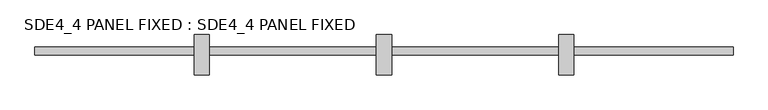
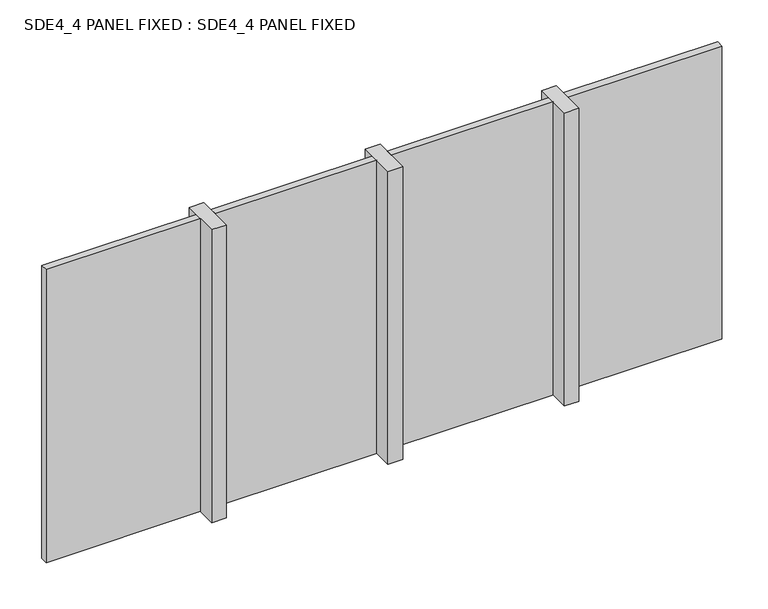
"""IFC4 building model written with IfcOpenShell, lengths in millimetres: plate geometry, SDE4_4 PANEL FIXED : SDE4_4 PANEL FIXED."""

from ifc_helpers import new_model, si_unit, origin, origin_with_axes, place, context, project, spatial, polyline, outline, extrude, source, transform, mapped, element, save


def sde4_4_panel_fixed_sde4_4_panel_fixed_a4a4073a(model_context):
    return source(origin(), model_context, "Body", "SweptSolid", [
        extrude(outline(polyline([(-1150.0, 132.5), (-1150.0, -132.5), (-1250.0, -132.5), (-1250.0, 132.5), (-1150.0, 132.5)])), origin_with_axes(), (0.0, 0.0, 1.0), 2110.0),
        extrude(outline(polyline([(50.0, 132.5), (50.0, -132.5), (-50.0, -132.5), (-50.0, 132.5), (50.0, 132.5)])), origin_with_axes(), (0.0, 0.0, 1.0), 2110.0),
        extrude(outline(polyline([(1250.0, 132.5), (1250.0, -132.5), (1150.0, -132.5), (1150.0, 132.5), (1250.0, 132.5)])), origin_with_axes(), (0.0, 0.0, 1.0), 2110.0),
        extrude(outline(polyline([(2299.0, 50.0), (2299.0, 0.0), (1250.0, 0.0), (1250.0, 50.0), (2299.0, 50.0)])), origin_with_axes(), (0.0, 0.0, 1.0), 2110.0),
        extrude(outline(polyline([(1150.0, 50.0), (1150.0, 0.0), (50.0, 0.0), (50.0, 50.0), (1150.0, 50.0)])), origin_with_axes(), (0.0, 0.0, 1.0), 2110.0),
        extrude(outline(polyline([(-50.0, 50.0), (-50.0, 0.0), (-1150.0, 0.0), (-1150.0, 50.0), (-50.0, 50.0)])), origin_with_axes(), (0.0, 0.0, 1.0), 2110.0),
        extrude(outline(polyline([(-1250.0, 50.0), (-1250.0, 0.0), (-2300.0, 0.0), (-2300.0, 50.0), (-1250.0, 50.0)])), origin_with_axes(), (0.0, 0.0, 1.0), 2110.0),
    ])


if __name__ == "__main__":
    model = new_model("IFC4")
    model_context = context("Model", 3, world=origin())
    ifc_project = project(units=[si_unit("LENGTHUNIT", "METRE", prefix="MILLI")], contexts=[model_context])
    site = spatial("IfcSite", under=ifc_project)
    building = spatial("IfcBuilding", under=site)
    placement = place(None, origin())
    sde4_4_panel_fixed_sde4_4_panel_fixed_shape = sde4_4_panel_fixed_sde4_4_panel_fixed_a4a4073a(model_context)
    element("IfcPlate", 1, ObjectType="SDE4_4 PANEL FIXED : SDE4_4 PANEL FIXED", at=placement, inside=building, context=model_context, shape_type="MappedRepresentation", body=[
        mapped(sde4_4_panel_fixed_sde4_4_panel_fixed_shape, transform((0.0, 0.0, 0.0), x_axis=(1.0, 0.0, 0.0), y_axis=(0.0, 1.0, 0.0), z_axis=(0.0, 0.0, 1.0))),
    ])
    save(model, "model.ifc")

# Revit data of these elements
# Type "SDE4_4 PANEL FIXED : SDE4_4 PANEL FIXED"
#   Type Mark = "CW-GLASS"
#   Analytic Construction = "<None>"
#   Glass = Glass
#   Frame = Aluminium
# Element 1 (IfcPlate, "SDE4_4 PANEL FIXED : SDE4_4 PANEL FIXED")
#   Materials on its faces: "Glass", "Aluminium"
# Materials
#   "Glass": class "Glass", colour RGB 0 128 192, transparency 0.9, Keynote = "L40", Cost = 0
#   "Aluminium": class "Unassigned", colour RGB 247 247 247, transparency 0, Cost = 0
